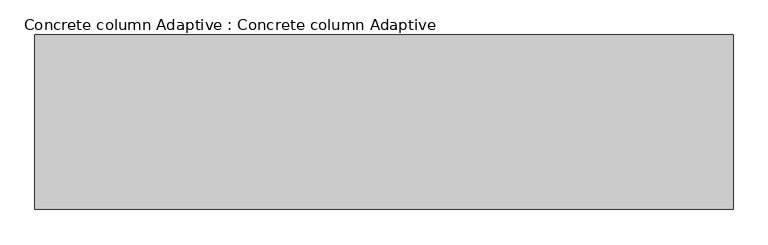
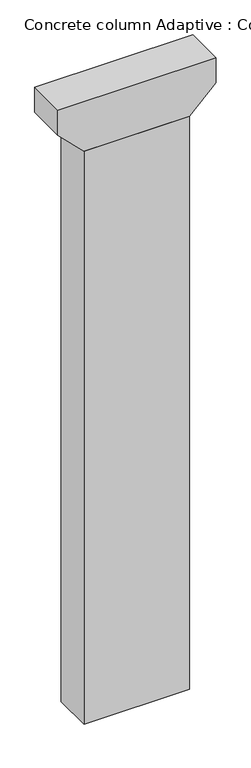
"""IFC4 building model written with IfcOpenShell, lengths in millimetres: proxy geometry, Concrete column Adaptive : Concrete column Adaptive."""

from ifc_helpers import new_model, si_unit, frame, origin, origin_with_axes, place, context, project, spatial, polyline, outline, extrude, source, transform, mapped, element, save


def concrete_column_adaptive_concrete_column_adaptive_a8665295(model_context):
    return source(origin(), model_context, "Body", "SweptSolid", [
        extrude(outline(polyline([(49912.0, 6000.0), (49912.0, -6000.0), (47912.0, -6000.0), (45912.0, -4000.0), (45912.0, 4000.0), (47912.0, 6000.0), (49912.0, 6000.0)])), frame((0.0, -1500.0, 0.0), z_axis=(0.0, 1.0, 0.0), x_axis=(0.0, 0.0, 1.0)), (0.0, 0.0, 1.0), 3000.0),
        extrude(outline(polyline([(-4000.0, -1500.0), (-4000.0, 1500.0), (4000.0, 1500.0), (4000.0, -1500.0), (-4000.0, -1500.0)])), origin_with_axes(), (0.0, 0.0, 1.0), 45912.0),
    ])


if __name__ == "__main__":
    model = new_model("IFC4")
    model_context = context("Model", 3, world=origin())
    ifc_project = project(units=[si_unit("LENGTHUNIT", "METRE", prefix="MILLI")], contexts=[model_context])
    site = spatial("IfcSite", under=ifc_project)
    building = spatial("IfcBuilding", under=site)
    placement = place(None, origin())
    concrete_column_adaptive_concrete_column_adaptive_shape = concrete_column_adaptive_concrete_column_adaptive_a8665295(model_context)
    element("IfcBuildingElementProxy", 1, Name="Concrete column Adaptive : Concrete column Adaptive", ObjectType="Concrete column Adaptive : Concrete column Adaptive", at=placement, inside=building, context=model_context, shape_type="MappedRepresentation", body=[
        mapped(concrete_column_adaptive_concrete_column_adaptive_shape, transform((0.0, 0.0, 0.0), x_axis=(1.0, 0.0, 0.0), y_axis=(0.0, 1.0, 0.0), z_axis=(0.0, 0.0, 1.0))),
    ])
    save(model, "model.ifc")

# Revit data of these elements
# Type "Concrete column Adaptive : Concrete column Adaptive"
#   Height [instance default] = 30000 mm
#   Default Elevation = 0
# Element 1 (IfcBuildingElementProxy, "Concrete column Adaptive : Concrete column Adaptive")
#   Height = 45912 mm
